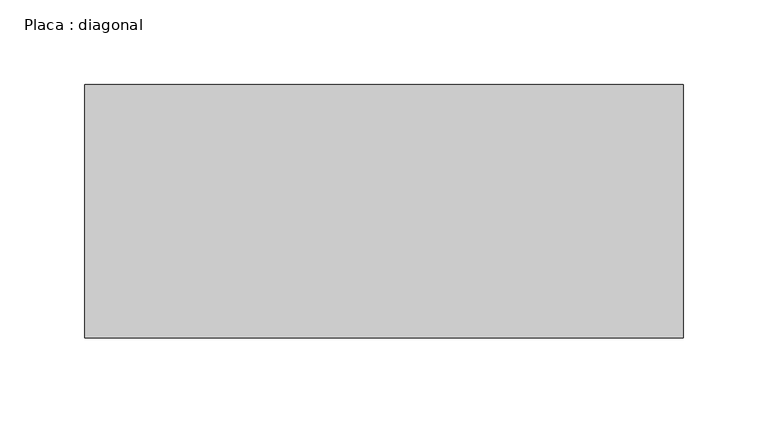
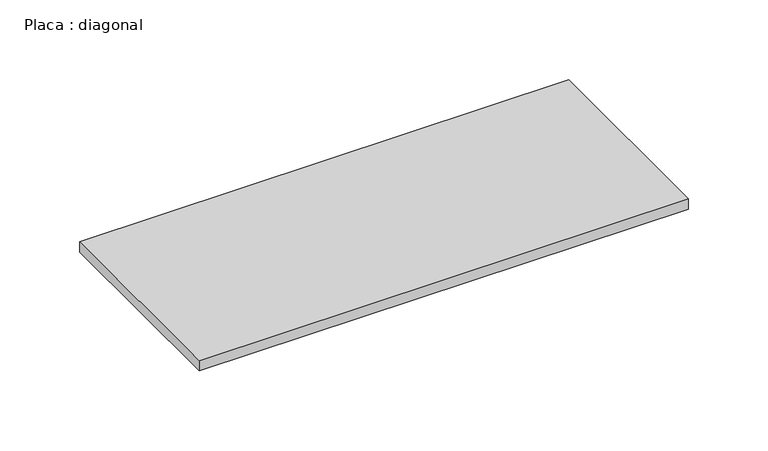
"""IFC4 building model written with IfcOpenShell, lengths in millimetres: beam geometry, Placa : diagonal."""

from ifc_helpers import new_model, si_unit, frame, origin, place, context, project, spatial, polyline, outline, extrude, source, transform, mapped, element, save


def placa_diagonal_9cc04f9e(model_context):
    return source(origin(), model_context, "Body", "SweptSolid", [
        extrude(outline(polyline([(177.4551585, 75.0), (177.4551585, -75.0), (-176.322012, -75.0), (-176.322012, 75.0), (177.4551585, 75.0)])), frame((0.0, 0.0, -4.0), z_axis=(0.0, 0.0, 1.0), x_axis=(1.0, 0.0, 0.0)), (0.0, 0.0, 1.0), 8.0),
    ])


if __name__ == "__main__":
    model = new_model("IFC4")
    model_context = context("Model", 3, world=origin())
    ifc_project = project(units=[si_unit("LENGTHUNIT", "METRE", prefix="MILLI")], contexts=[model_context])
    site = spatial("IfcSite", under=ifc_project)
    building = spatial("IfcBuilding", under=site)
    placement = place(None, origin())
    placa_diagonal_shape = placa_diagonal_9cc04f9e(model_context)
    element("IfcBeam", 1, ObjectType="Placa : diagonal", at=placement, inside=building, context=model_context, shape_type="MappedRepresentation", body=[
        mapped(placa_diagonal_shape, transform((0.0, 0.0, 0.0), x_axis=(1.0, 0.0, 0.0), y_axis=(0.0, 1.0, 0.0), z_axis=(0.0, 0.0, 1.0))),
    ])
    save(model, "model.ifc")

# Revit data of these elements
# Type "Placa : diagonal"
#   W = 0
#   Length [instance default] = 1.50 m
#   b = 0.15 m
#   d = 0.008 m
#   A = 0 m²
#   Structural Material [instance default] = Aço, 45-345
# Element 1 (IfcBeam, "Placa : diagonal")
#   Materials on its faces: "Aço, 45-345"
# Materials
#   "Aço, 45-345": class "Metal", colour RGB 247 247 247, transparency 0, Description = "Aço 345 MPa", Cost = 0
